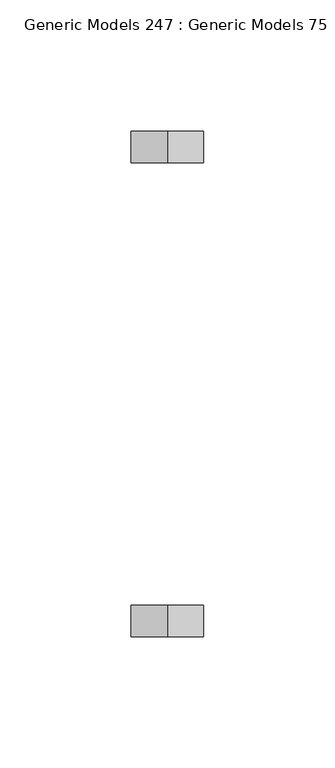
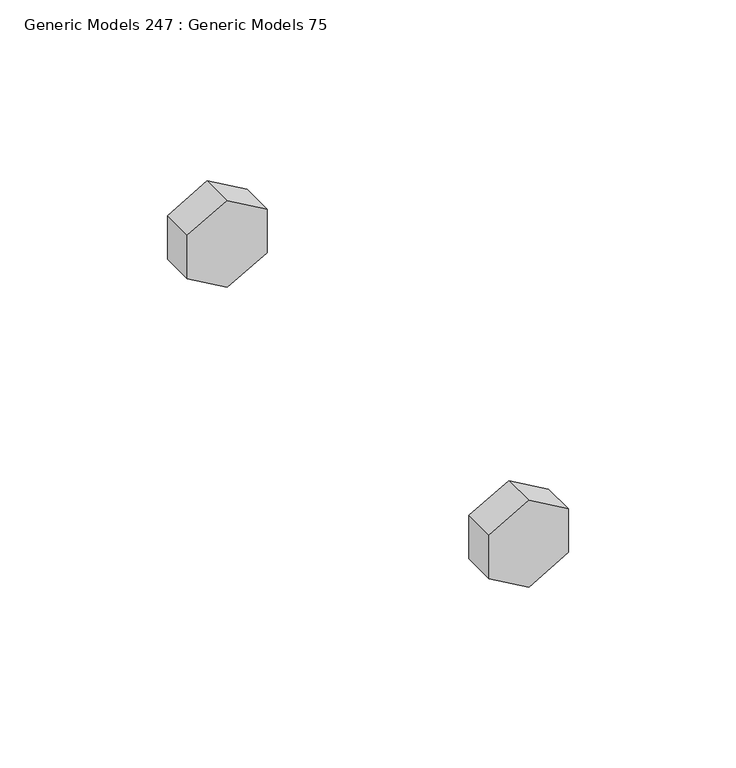
"""IFC4 building model written with IfcOpenShell, lengths in millimetres: proxy geometry, Generic Models 247 : Generic Models 75."""

from ifc_helpers import new_model, si_unit, frame, origin, place, context, project, spatial, polyline, outline, extrude, source, transform, mapped, element, save


def generic_models_247_generic_models_75_025838be(model_context):
    return source(origin(), model_context, "Body", "SweptSolid", [
        extrude(outline(polyline([(269374.7462802, 31975.9942029), (269358.9097067, 31975.9942029), (269350.99142, 31989.7090778), (269358.9097067, 32003.4239528), (269374.7462802, 32003.4239528), (269382.664567, 31989.7090778), (269374.7462802, 31975.9942029)])), frame((0.0, 35373.9582942, 0.0), z_axis=(0.0, 1.0, 0.0), x_axis=(0.0, 0.0, 1.0)), (0.0, 0.0, 1.0), 11.90625),
        extrude(outline(polyline([(269374.7462802, 31975.9942029), (269358.9097067, 31975.9942029), (269350.99142, 31989.7090778), (269358.9097067, 32003.4239528), (269374.7462802, 32003.4239528), (269382.664567, 31989.7090778), (269374.7462802, 31975.9942029)])), frame((0.0, 35193.7770442, 0.0), z_axis=(0.0, 1.0, 0.0), x_axis=(0.0, 0.0, 1.0)), (0.0, 0.0, 1.0), 11.90625),
    ])


if __name__ == "__main__":
    model = new_model("IFC4")
    model_context = context("Model", 3, world=origin())
    ifc_project = project(units=[si_unit("LENGTHUNIT", "METRE", prefix="MILLI")], contexts=[model_context])
    site = spatial("IfcSite", under=ifc_project)
    building = spatial("IfcBuilding", under=site)
    placement = place(None, origin())
    generic_models_247_generic_models_75_shape = generic_models_247_generic_models_75_025838be(model_context)
    element("IfcBuildingElementProxy", 1, Name="Generic Models 247 : Generic Models 75", ObjectType="Generic Models 247 : Generic Models 75", at=placement, inside=building, context=model_context, shape_type="MappedRepresentation", body=[
        mapped(generic_models_247_generic_models_75_shape, transform((0.0, 0.0, 0.0), x_axis=(1.0, 0.0, 0.0), y_axis=(0.0, 1.0, 0.0), z_axis=(0.0, 0.0, 1.0))),
    ])
    save(model, "model.ifc")

# Revit data of these elements
# Element 1 (IfcBuildingElementProxy, "Generic Models 247 : Generic Models 75")
#   Materials on its faces: "3/4\" GALV. THRU BOLTS"
# Materials
#   "3/4\" GALV. THRU BOLTS": class "Generic", colour RGB 105 69 171, transparency 0, Cost = 0
